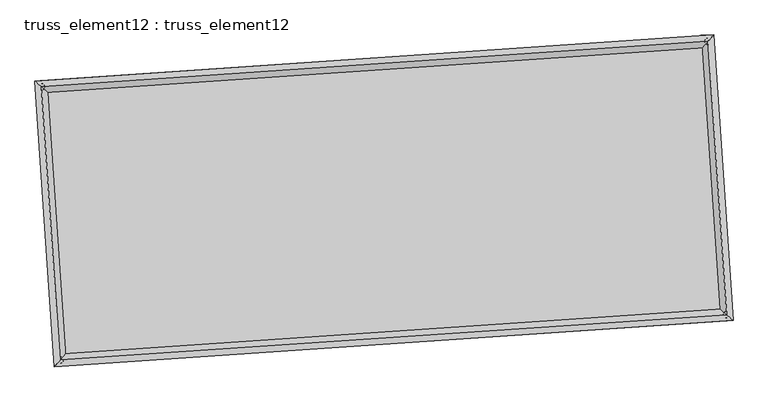
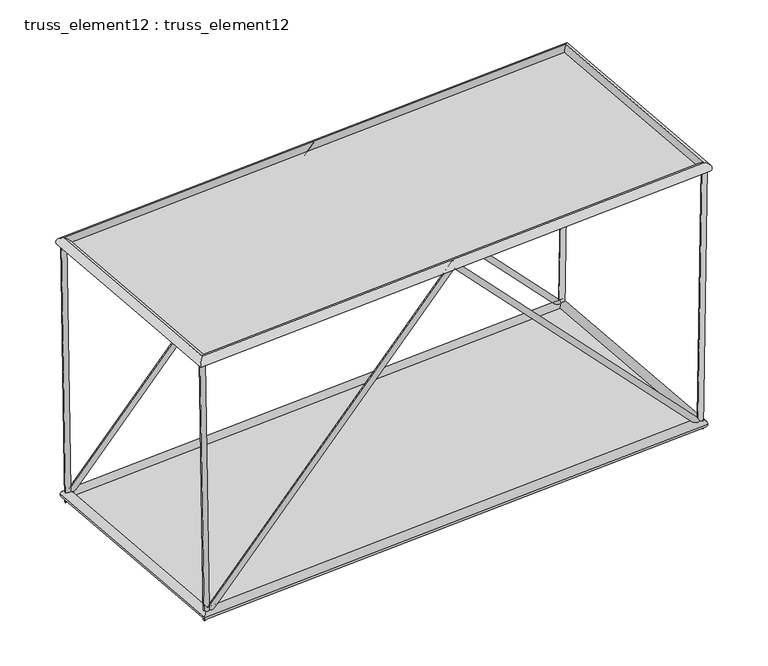
"""IFC4 building model written with IfcOpenShell, lengths in millimetres: plate geometry, truss_element12 : truss_element12."""

from ifc_helpers import new_model, si_unit, frame, origin, origin_with_axes, place, context, project, spatial, polyline, circle_curve, ellipse_curve, outline, extrude, source, transform, mapped, element, save
from ifc_brep_helpers import plane_surface, cylinder_surface, advanced_brep


def truss_element12_truss_element12_1bbcfac7(model_context):
    return source(origin(), model_context, "Body", "SolidModel", [
        advanced_brep(
        [(-3746.2779315, 2270.677949, 5000.1488437), (-3845.3680681, 2257.3176242, 4998.522018), (-3666.9216571, 2276.0889517, 122.1113591), (-3762.0652257, 2262.9977284, -122.1113591), (1064.4228838, 2598.7013505, 5071.4427935), (1064.8605805, 2592.1274502, 4927.2050495), (5794.3942317, 2921.2201164, 122.1016693), (5890.3667453, 2921.1603721, -122.1016693), (5875.1134246, 2926.7240513, 5000.1397912), (5975.0995037, 2926.9379768, 4998.4850331)],
        [
            (0, 1, circle_curve(frame((-3795.8229998, 2263.9977866, 4999.3354308), z_axis=(-0.016265911675968303, -0.0011091106846651264, 0.9998670861623754), x_axis=(-0.1336035338535352, 0.9910342788842121, -0.0010741593443196402)), 50.0)),
            (1, 0, circle_curve(frame((-3795.8229998, 2263.9977866, 4999.3354308), z_axis=(-0.016265911675968303, -0.0011091106846651264, 0.9998670861623754), x_axis=(-0.1336035338535352, 0.9910342788842121, -0.0010741593443196402)), 50.0)),
            (0, 2),
            (2, 3, ellipse_curve(frame((-3714.4934414, 2269.54334, 0.0), z_axis=(-0.9287646394568875, -0.06332893019963927, 0.36522005845009003), x_axis=(0.36437398822915085, 0.02484527714214224, 0.9309212151979955)), 131.4582279, 50.0)),
            (3, 1),
            (3, 2, ellipse_curve(frame((-3714.4934414, 2269.54334, 0.0), z_axis=(-0.9287646394568875, -0.06332893019963927, 0.36522005845009003), x_axis=(0.36437398822915085, 0.02484527714214224, 0.9309212151979955)), 131.4582279, 50.0)),
            (2, 4),
            (4, 5, ellipse_curve(frame((1064.6417322, 2595.4144003, 4999.3239215), z_axis=(-0.9976833934171915, -0.06802823804748175, 7.299118212849759e-05), x_axis=(-7.282209046969254e-05, -4.9654615264680074e-06, -0.9999999973361436)), 72.2759091, 50.0)),
            (5, 3),
            (5, 4, ellipse_curve(frame((1064.6417322, 2595.4144003, 4999.3239215), z_axis=(-0.9976833934171915, -0.06802823804748175, 7.299118212849759e-05), x_axis=(-7.282209046969254e-05, -4.9654615264680074e-06, -0.9999999973361436)), 72.2759091, 50.0)),
            (4, 6),
            (6, 7, ellipse_curve(frame((5842.3804885, 2921.1902443, 0.0), z_axis=(-0.9288422213363277, -0.06333422021308223, -0.3650217862169288), x_axis=(-0.3641761753142233, -0.02483178903143046, 0.930998977221244)), 131.4368172, 50.0)),
            (7, 5),
            (7, 6, ellipse_curve(frame((5842.3804885, 2921.1902443, 0.0), z_axis=(-0.9288422213363277, -0.06333422021308223, -0.3650217862169288), x_axis=(-0.3641761753142233, -0.02483178903143046, 0.930998977221244)), 131.4368172, 50.0)),
            (8, 9, circle_curve(frame((5925.1064641, 2926.8310141, 4999.3124122), z_axis=(0.016545195126702994, 0.0011281539615151874, 0.9998624824378893), x_axis=(-0.0021576295961431924, 0.9999970754228623, -0.0010926025114963022)), 50.0)),
            (9, 8, circle_curve(frame((5925.1064641, 2926.8310141, 4999.3124122), z_axis=(0.016545195126702994, 0.0011281539615151874, 0.9998624824378893), x_axis=(-0.0021576295961431924, 0.9999970754228623, -0.0010926025114963022)), 50.0)),
            (6, 8),
            (9, 7),
        ],
        [
            plane_surface(frame((-3795.8229998, 2313.9977559, 4999.3908937), z_axis=(-0.016265911675968123, -0.0011091106846617949, 0.9998670861623753), x_axis=(0.9998677013072027, -1.8043083511720685e-05, 0.01626590166875275))),
            cylinder_surface(frame((-3795.8229998, 2263.9977866, 4999.3354308), z_axis=(-0.016265911675968303, -0.0011091106846651264, 0.9998670861623754), x_axis=(-0.1336035338535352, 0.9910342788842121, -0.0010741593443196402)), 50.0),
            cylinder_surface(frame((-3714.4934414, 2269.54334, 0.0), z_axis=(-0.6902434140818179, -0.04706507454537663, -0.7220449487910807), x_axis=(-0.020419087296308105, 0.9987518960405878, -0.045581915595078945)), 50.0),
            cylinder_surface(frame((1064.6417322, 2595.4144003, 4999.3239215), z_axis=(-0.6901382450820931, -0.04705790347107014, 0.7221459384334419), x_axis=(-0.11534841177711228, 0.9922790262643878, -0.045574970502419106)), 50.0),
            plane_surface(frame((5925.1064641, 2876.8310459, 4999.3688276), z_axis=(0.01654519512670156, 0.0011281539615101215, 0.9998624824378892), x_axis=(0.9998631188908906, -1.8668082734762968e-05, -0.016545184595020874))),
            cylinder_surface(frame((5842.3804885, 2921.1902443, 0.0), z_axis=(-0.016545195126702994, -0.0011281539615151874, -0.9998624824378893), x_axis=(-0.0021576295961431924, 0.9999970754228623, -0.0010926025114963022)), 50.0),
        ],
        [
            (0, [[1, 2]]),
            (1, [[-1, 3, 4, 5]]),
            (1, [[-2, -5, 6, -3]]),
            (2, [[-4, 7, 8, 9]]),
            (2, [[-6, -9, 10, -7]]),
            (3, [[-8, 11, 12, 13]]),
            (3, [[-10, -13, 14, -11]]),
            (4, [[15, 16]]),
            (5, [[-12, 17, -16, 18]]),
            (5, [[-14, -18, -15, -17]]),
        ],
    ),
        advanced_brep(
        [(-3474.1649786, -1720.0556353, 5000.1488437), (-3573.2551151, -1733.4159601, 4998.522018), (-3394.8087042, -1714.6446326, 122.1113591), (-3489.9522728, -1727.7358559, -122.1113591), (1336.5358367, -1392.0322338, 5071.4427935), (1336.9735335, -1398.6061341, 4927.2050495), (6066.5071846, -1069.5134679, 122.1016693), (6162.4796982, -1069.5732122, -122.1016693), (6147.2263775, -1064.009533, 5000.1397912), (6247.2124566, -1063.7956075, 4998.4850331)],
        [
            (0, 1, circle_curve(frame((-3523.7100469, -1726.7357977, 4999.3354308), z_axis=(-0.01626591167596829, -0.0011091106846651422, 0.9998670861623754), x_axis=(-0.13360353385353582, 0.991034278884212, -0.0010741593443196332)), 50.0)),
            (1, 0, circle_curve(frame((-3523.7100469, -1726.7357977, 4999.3354308), z_axis=(-0.01626591167596829, -0.0011091106846651422, 0.9998670861623754), x_axis=(-0.13360353385353582, 0.991034278884212, -0.0010741593443196332)), 50.0)),
            (0, 2),
            (2, 3, ellipse_curve(frame((-3442.3804885, -1721.1902443, 0.0), z_axis=(-0.9287646394568875, -0.06332893019963957, 0.36522005845009003), x_axis=(0.36437398822915085, 0.02484527714214235, 0.9309212151979955)), 131.4582279, 50.0)),
            (3, 1),
            (3, 2, ellipse_curve(frame((-3442.3804885, -1721.1902443, 0.0), z_axis=(-0.9287646394568875, -0.06332893019963957, 0.36522005845009003), x_axis=(0.36437398822915085, 0.02484527714214235, 0.9309212151979955)), 131.4582279, 50.0)),
            (2, 4),
            (4, 5, ellipse_curve(frame((1336.7546851, -1395.319184, 4999.3239215), z_axis=(-0.9976833934171915, -0.06802823804748206, 7.299118212825683e-05), x_axis=(-7.282209046923131e-05, -4.965461526419962e-06, -0.9999999973361436)), 72.2759091, 50.0)),
            (5, 3),
            (5, 4, ellipse_curve(frame((1336.7546851, -1395.319184, 4999.3239215), z_axis=(-0.9976833934171915, -0.06802823804748206, 7.299118212825683e-05), x_axis=(-7.282209046923131e-05, -4.965461526419962e-06, -0.9999999973361436)), 72.2759091, 50.0)),
            (4, 6),
            (6, 7, ellipse_curve(frame((6114.4934414, -1069.54334, 0.0), z_axis=(-0.9288422213363275, -0.06333422021308248, -0.3650217862169293), x_axis=(-0.3641761753142236, -0.024831789031430622, 0.930998977221244)), 131.4368172, 50.0)),
            (7, 5),
            (7, 6, ellipse_curve(frame((6114.4934414, -1069.54334, 0.0), z_axis=(-0.9288422213363275, -0.06333422021308248, -0.3650217862169293), x_axis=(-0.3641761753142236, -0.024831789031430622, 0.930998977221244)), 131.4368172, 50.0)),
            (8, 9, circle_curve(frame((6197.2194171, -1063.9025702, 4999.3124122), z_axis=(0.016545195126702262, 0.0011281539615151067, 0.9998624824378893), x_axis=(-0.0021576295961430463, 0.9999970754228623, -0.0010926025114962256)), 50.0)),
            (9, 8, circle_curve(frame((6197.2194171, -1063.9025702, 4999.3124122), z_axis=(0.016545195126702262, 0.0011281539615151067, 0.9998624824378893), x_axis=(-0.0021576295961430463, 0.9999970754228623, -0.0010926025114962256)), 50.0)),
            (6, 8),
            (9, 7),
        ],
        [
            plane_surface(frame((-3523.7100469, -1676.7358284, 4999.3908937), z_axis=(-0.016265911675968123, -0.001109110684661801, 0.9998670861623753), x_axis=(0.9998677013072027, -1.8043083511720685e-05, 0.01626590166875275))),
            cylinder_surface(frame((-3523.7100469, -1726.7357977, 4999.3354308), z_axis=(-0.01626591167596829, -0.0011091106846651422, 0.9998670861623754), x_axis=(-0.13360353385353582, 0.991034278884212, -0.0010741593443196332)), 50.0),
            cylinder_surface(frame((-3442.3804885, -1721.1902443, 0.0), z_axis=(-0.690243414081818, -0.04706507454537685, -0.7220449487910808), x_axis=(-0.020419087296308168, 0.9987518960405878, -0.045581915595079174)), 50.0),
            cylinder_surface(frame((1336.7546851, -1395.319184, 4999.3239215), z_axis=(-0.6901382450820935, -0.0470579034710704, 0.7221459384334415), x_axis=(-0.1153484117771128, 0.9922790262643877, -0.04557497050241935)), 50.0),
            plane_surface(frame((6197.2194171, -1113.9025384, 4999.3688276), z_axis=(0.016545195126701558, 0.001128153961510126, 0.9998624824378892), x_axis=(0.9998631188908906, -1.866808273431888e-05, -0.016545184595020874))),
            cylinder_surface(frame((6114.4934414, -1069.54334, 0.0), z_axis=(-0.016545195126702262, -0.0011281539615151067, -0.9998624824378893), x_axis=(-0.0021576295961430463, 0.9999970754228623, -0.0010926025114962256)), 50.0),
        ],
        [
            (0, [[1, 2]]),
            (1, [[-1, 3, 4, 5]]),
            (1, [[-2, -5, 6, -3]]),
            (2, [[-4, 7, 8, 9]]),
            (2, [[-6, -9, 10, -7]]),
            (3, [[-8, 11, 12, 13]]),
            (3, [[-10, -13, 14, -11]]),
            (4, [[15, 16]]),
            (5, [[-12, 17, -16, 18]]),
            (5, [[-14, -18, -15, -17]]),
        ],
    ),
        advanced_brep(
        [(-3523.7160635, -1726.7424662, 4909.335431), (-3523.7040302, -1726.7291292, 5089.3354306), (-3795.8161337, 2263.9919966, 5089.3354306), (-3795.8298659, 2264.0035767, 4909.335431), (5925.1008717, 2926.8243745, 5089.312412), (5925.1120565, 2926.8376536, 4909.3124124), (6197.2129752, -1063.8967513, 5089.312412), (6197.2258589, -1063.9083892, 4909.3124124)],
        [
            (0, 1, ellipse_curve(frame((-3523.7100469, -1726.7357977, 4999.3354308), z_axis=(-0.7535719234034886, 0.6573654662782159, 1.670510786331496e-06), x_axis=(-0.657365466276113, -0.7535719234053231, 1.6705107863314674e-06)), 127.2792206, 90.0)),
            (1, 2),
            (2, 3, ellipse_curve(frame((-3795.8229998, 2263.9977866, 4999.3354308), z_axis=(-0.657365466276113, -0.7535719234053231, 1.6705107863314422e-06), x_axis=(0.7535719234034887, -0.6573654662782157, -1.6705107863314712e-06)), 127.2792206, 90.0)),
            (3, 0),
            (1, 0, ellipse_curve(frame((-3523.7100469, -1726.7357977, 4999.3354308), z_axis=(-0.7535719234034886, 0.6573654662782159, 1.670510786331496e-06), x_axis=(-0.657365466276113, -0.7535719234053231, 1.6705107863314674e-06)), 127.2792206, 90.0)),
            (3, 2, ellipse_curve(frame((-3795.8229998, 2263.9977866, 4999.3354308), z_axis=(-0.657365466276113, -0.7535719234053231, 1.6705107863314422e-06), x_axis=(0.7535719234034887, -0.6573654662782157, -1.6705107863314712e-06)), 127.2792206, 90.0)),
            (2, 4),
            (4, 5, ellipse_curve(frame((5925.1064641, 2926.8310141, 4999.3124122), z_axis=(-0.7535719234034886, 0.6573654662782158, 1.670510786331446e-06), x_axis=(-0.657365466276113, -0.7535719234053229, 1.6705107863314674e-06)), 127.2792206, 90.0)),
            (5, 3),
            (5, 4, ellipse_curve(frame((5925.1064641, 2926.8310141, 4999.3124122), z_axis=(-0.7535719234034886, 0.6573654662782158, 1.670510786331446e-06), x_axis=(-0.657365466276113, -0.7535719234053229, 1.6705107863314674e-06)), 127.2792206, 90.0)),
            (4, 6),
            (6, 7, ellipse_curve(frame((6197.2194171, -1063.9025702, 4999.3124122), z_axis=(0.6573654662761127, 0.7535719234053232, -1.6705107863314917e-06), x_axis=(-0.7535719234034888, 0.6573654662782156, 1.6705107863314714e-06)), 127.2792206, 90.0)),
            (7, 5),
            (7, 6, ellipse_curve(frame((6197.2194171, -1063.9025702, 4999.3124122), z_axis=(0.6573654662761127, 0.7535719234053232, -1.6705107863314917e-06), x_axis=(-0.7535719234034888, 0.6573654662782156, 1.6705107863314714e-06)), 127.2792206, 90.0)),
            (6, 1),
            (0, 7),
        ],
        [
            cylinder_surface(frame((-3523.7100469, -1726.7357977, 4999.3354308), z_axis=(0.06802823822869979, -0.9976833960748768, 0.0), x_axis=(-0.9976833935077207, -0.06802823805365518, 7.173725476019441e-05)), 90.0),
            cylinder_surface(frame((-3795.8229998, 2263.9977866, 4999.3354308), z_axis=(-0.9976833960720926, -0.06802823822851069, 2.3624590101204896e-06), x_axis=(-0.06802823790147983, 0.9976833936851698, 6.937479575575899e-05)), 90.0),
            cylinder_surface(frame((5925.1064641, 2926.8310141, 4999.3124122), z_axis=(-0.06802823822870002, 0.9976833960748767, 0.0), x_axis=(0.9976833938347516, 0.0680282380759544, 6.701233675132358e-05)), 90.0),
            cylinder_surface(frame((6197.2194171, -1063.9025702, 4999.3124122), z_axis=(0.9976833960720927, 0.0680282382285108, -2.362459010120525e-06), x_axis=(0.0680282382285108, -0.9976833936628708, 6.937479575575899e-05)), 90.0),
        ],
        [
            (0, [[1, 2, 3, 4]]),
            (0, [[5, -4, 6, -2]]),
            (1, [[-3, 7, 8, 9]]),
            (1, [[-6, -9, 10, -7]]),
            (2, [[-8, 11, 12, 13]]),
            (2, [[-10, -13, 14, -11]]),
            (3, [[-12, 15, -1, 16]]),
            (3, [[-14, -16, -5, -15]]),
        ],
    ),
        advanced_brep(
        [(-3358.7115243, -1625.2761972, 0.0), (-3526.0494527, -1817.1042913, 0.0), (-3810.4074885, 2353.2123043, 0.0), (-3618.5793943, 2185.8743758, 0.0), (5926.0494527, 3017.1042913, 0.0), (5758.7115243, 2825.2761972, 0.0), (6210.4074885, -1153.2123043, 0.0), (6018.5793943, -985.8743758, 0.0)],
        [
            (0, 1, ellipse_curve(frame((-3442.3804885, -1721.1902443, 0.0), z_axis=(-0.7535719234054563, 0.6573654662780828, 0.0), x_axis=(-0.6573654662780828, -0.7535719234054562, 0.0)), 127.2792206, 90.0)),
            (1, 2),
            (2, 3, ellipse_curve(frame((-3714.4934414, 2269.54334, 0.0), z_axis=(-0.6573654662780828, -0.7535719234054563, 0.0), x_axis=(0.7535719234054564, -0.6573654662780826, 0.0)), 127.2792206, 90.0)),
            (3, 0),
            (1, 0, ellipse_curve(frame((-3442.3804885, -1721.1902443, 0.0), z_axis=(-0.7535719234054563, 0.6573654662780828, 0.0), x_axis=(-0.6573654662780828, -0.7535719234054562, 0.0)), 127.2792206, 90.0)),
            (3, 2, ellipse_curve(frame((-3714.4934414, 2269.54334, 0.0), z_axis=(-0.6573654662780828, -0.7535719234054563, 0.0), x_axis=(0.7535719234054564, -0.6573654662780826, 0.0)), 127.2792206, 90.0)),
            (2, 4),
            (4, 5, ellipse_curve(frame((5842.3804885, 2921.1902443, 0.0), z_axis=(-0.7535719234054562, 0.6573654662780827, 0.0), x_axis=(-0.6573654662780829, -0.7535719234054562, 0.0)), 127.2792206, 90.0)),
            (5, 3),
            (5, 4, ellipse_curve(frame((5842.3804885, 2921.1902443, 0.0), z_axis=(-0.7535719234054562, 0.6573654662780827, 0.0), x_axis=(-0.6573654662780829, -0.7535719234054562, 0.0)), 127.2792206, 90.0)),
            (4, 6),
            (6, 7, ellipse_curve(frame((6114.4934414, -1069.54334, 0.0), z_axis=(0.6573654662780828, 0.7535719234054563, 0.0), x_axis=(-0.7535719234054563, 0.6573654662780827, 0.0)), 127.2792206, 90.0)),
            (7, 5),
            (7, 6, ellipse_curve(frame((6114.4934414, -1069.54334, 0.0), z_axis=(0.6573654662780828, 0.7535719234054563, 0.0), x_axis=(-0.7535719234054563, 0.6573654662780827, 0.0)), 127.2792206, 90.0)),
            (6, 1),
            (0, 7),
        ],
        [
            cylinder_surface(frame((-3442.3804885, -1721.1902443, 0.0), z_axis=(0.0680282382286984, -0.9976833960748769, 0.0), x_axis=(-0.9976833960748769, -0.0680282382286984, 0.0)), 90.0),
            cylinder_surface(frame((-3714.4934414, 2269.54334, 0.0), z_axis=(-0.9976833960748769, -0.06802823822869901, 0.0), x_axis=(-0.06802823822869901, 0.9976833960748769, 0.0)), 90.0),
            cylinder_surface(frame((5842.3804885, 2921.1902443, 0.0), z_axis=(-0.06802823822869834, 0.9976833960748769, 0.0), x_axis=(0.9976833960748769, 0.06802823822869834, 0.0)), 90.0),
            cylinder_surface(frame((6114.4934414, -1069.54334, 0.0), z_axis=(0.9976833960748768, 0.0680282382286991, 0.0), x_axis=(0.0680282382286991, -0.9976833960748768, 0.0)), 90.0),
        ],
        [
            (0, [[1, 2, 3, 4]]),
            (0, [[5, -4, 6, -2]]),
            (1, [[-3, 7, 8, 9]]),
            (1, [[-6, -9, 10, -7]]),
            (2, [[-8, 11, 12, 13]]),
            (2, [[-10, -13, 14, -11]]),
            (3, [[-12, 15, -1, 16]]),
            (3, [[-14, -16, -5, -15]]),
        ],
    ),
        extrude(outline(polyline([(-3442.3804885, -1721.1902443), (-3714.4934414, 2269.54334), (5842.3804885, 2921.1902443), (6114.4934414, -1069.54334), (-3442.3804885, -1721.1902443)])), origin_with_axes(), (0.0, 0.0, 1.0), 20.0),
        extrude(outline(polyline([(-2000.0, 4871.7506486), (2000.0, 4871.7506486), (2000.0, -4871.7506486), (-2000.0, -4871.7506487), (-2000.0, 4871.7506486)])), frame((1200.6982086, 600.0476082, 4999.3239215), z_axis=(2.3569861283047194e-06, 1.6071392434601366e-07, 0.9999999999972095), x_axis=(-0.06802823822869873, 0.9976833960748768, 0.0)), (0.0, 0.0, 1.0), 20.0),
    ])


if __name__ == "__main__":
    model = new_model("IFC4")
    model_context = context("Model", 3, world=origin())
    ifc_project = project(units=[si_unit("LENGTHUNIT", "METRE", prefix="MILLI")], contexts=[model_context])
    site = spatial("IfcSite", under=ifc_project)
    building = spatial("IfcBuilding", under=site)
    placement = place(None, origin())
    truss_element12_truss_element12_shape = truss_element12_truss_element12_1bbcfac7(model_context)
    element("IfcPlate", 1, ObjectType="truss_element12 : truss_element12", at=placement, inside=building, context=model_context, shape_type="MappedRepresentation", body=[
        mapped(truss_element12_truss_element12_shape, transform((0.0, 0.0, 0.0), x_axis=(1.0, 0.0, 0.0), y_axis=(0.0, 1.0, 0.0), z_axis=(0.0, 0.0, 1.0))),
    ])
    save(model, "model.ifc")

# Revit data of these elements
# Type "truss_element12 : truss_element12"
#   steellbar1 = 90 mm
#   steelbar2 = 50 mm
#   offset1 = 5000 mm
#   M = Default Roof
# Element 1 (IfcPlate, "truss_element12 : truss_element12")
#   Materials on its faces: "Default Roof"
# Materials
#   "Default Roof": class "Miscellaneous", colour RGB 0 127 0, transparency 0, Comments = "Rendering appearance not upgraded Rendering appearance not upgraded ", Cost = 0
